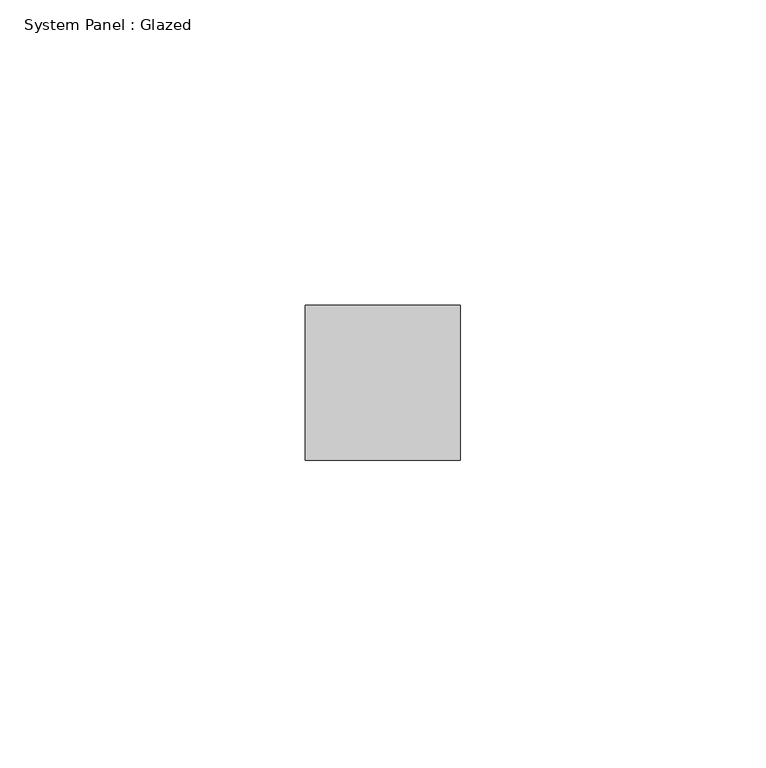
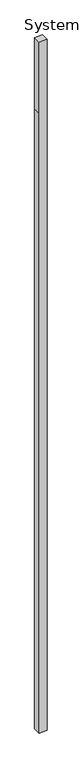
"""IFC4 building model written with IfcOpenShell, lengths in millimetres: plate geometry, System Panel : Glazed."""

from ifc_helpers import new_model, si_unit, frame, origin, place, context, project, spatial, polyline, outline, extrude, source, transform, mapped, element, save


def system_panel_glazed_99e16266(model_context):
    return source(origin(), model_context, "Body", "SweptSolid", [
        extrude(outline(polyline([(0.0, -12.7), (0.0, 12.7), (2101.85, 12.7), (2343.15, 12.7), (2343.15, -12.7), (2101.85, -12.7), (0.0, -12.7)])), frame((0.0, 19.05, 0.0), z_axis=(0.0, 1.0, 0.0), x_axis=(0.0, 0.0, 1.0)), (0.0, 0.0, 1.0), 25.4),
    ])


if __name__ == "__main__":
    model = new_model("IFC4")
    model_context = context("Model", 3, world=origin())
    ifc_project = project(units=[si_unit("LENGTHUNIT", "METRE", prefix="MILLI")], contexts=[model_context])
    site = spatial("IfcSite", under=ifc_project)
    building = spatial("IfcBuilding", under=site)
    placement = place(None, origin())
    system_panel_glazed_shape = system_panel_glazed_99e16266(model_context)
    element("IfcPlate", 1, ObjectType="System Panel : Glazed", at=placement, inside=building, context=model_context, shape_type="MappedRepresentation", body=[
        mapped(system_panel_glazed_shape, transform((0.0, 0.0, 0.0), x_axis=(1.0, 0.0, 0.0), y_axis=(0.0, 1.0, 0.0), z_axis=(0.0, 0.0, 1.0))),
    ])
    save(model, "model.ifc")

# Revit data of these elements
# Element 1 (IfcPlate, "System Panel : Glazed")
#   Materials on its faces: "Glass"
# Materials
#   "Glass": class "Glass", colour RGB 0 128 192, transparency 0.75, Cost = 0
